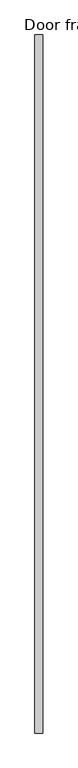
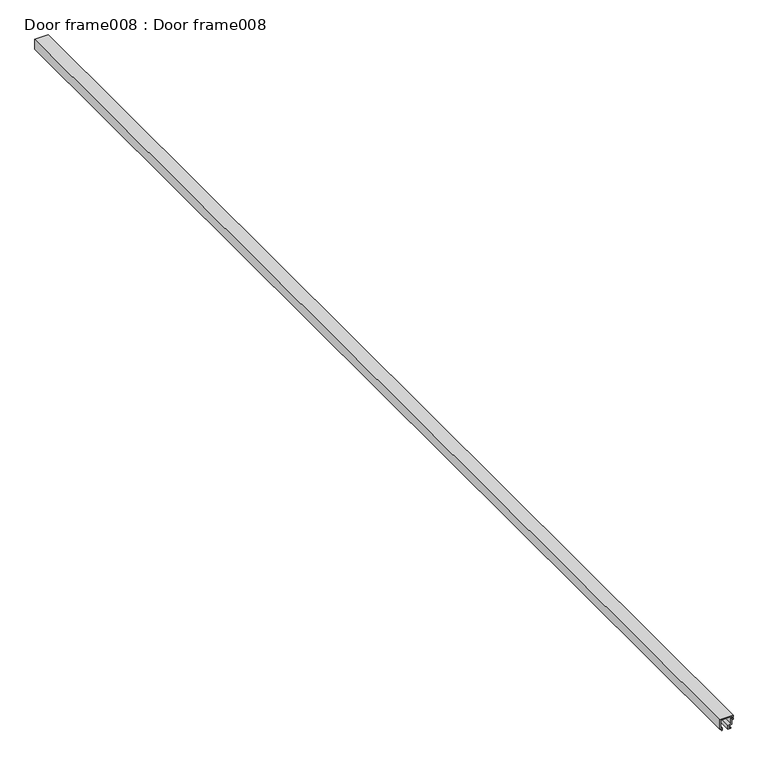
"""IFC4 building model written with IfcOpenShell, lengths in millimetres: proxy geometry, Door frame008 : Door frame008."""

import ifcopenshell
import ifcopenshell.guid

model = None  # the IFC model being written
_history = None  # IfcOwnerHistory: only IFC2X3 demands one
_inside = {}  # id of a spatial element -> (the spatial element, [elements in it])
_under = {}  # id of a project, library or spatial element -> (it, [spatial elements below it])
_declared = {}  # id of a project -> (the project, [libraries it declares])
_typed = {}  # id of a type object -> (the type object, [elements of that type])
_made_of = {}  # id of a material, layer set ... -> (it, [elements and type objects made of it])


def new_model(schema):
    """Start an empty IFC model of exactly this schema.

    Asked for "IFC4X3", IfcOpenShell would pick the latest addendum, in which some entities
    have other attributes; the version numbers below select the first issue.
    IFC2X3 requires an IfcOwnerHistory on every rooted entity: one is made here for all.
    """
    global model, _history
    if schema == "IFC4X3":
        model = ifcopenshell.file(schema_version=(4, 3, 0, 0))
    else:
        model = ifcopenshell.file(schema=schema)
    _inside.clear()
    _under.clear()
    _declared.clear()
    _typed.clear()
    _made_of.clear()
    _history = None
    if model.schema == "IFC2X3":
        org = make("IfcOrganization", Name="unknown")
        user = make(
            "IfcPersonAndOrganization",
            ThePerson=make("IfcPerson", FamilyName="unknown"),
            TheOrganization=org,
        )
        app = make(
            "IfcApplication",
            ApplicationDeveloper=org,
            Version="unknown",
            ApplicationFullName="unknown",
            ApplicationIdentifier="unknown",
        )
        _history = make(
            "IfcOwnerHistory",
            OwningUser=user,
            OwningApplication=app,
            ChangeAction="ADDED",
            CreationDate=0,
        )
    return model


def make(cls, **values):
    """One entity of the class cls with the attributes given. An attribute that is None is left unset."""
    return model.create_entity(
        cls, **{name: value for name, value in values.items() if value is not None}
    )


def rooted(cls, **values):
    """An entity with a GlobalId (a new one), such as an element, a storey or a relation."""
    return make(cls, GlobalId=ifcopenshell.guid.new(), OwnerHistory=_history, **values)


def si_unit(unit_type, name, prefix=None):
    """IfcSIUnit, for example si_unit("LENGTHUNIT", "METRE", prefix="MILLI")."""
    return make("IfcSIUnit", UnitType=unit_type, Prefix=prefix, Name=name)


def assignment(units):
    """IfcUnitAssignment: the units of a project."""
    return None if units is None else make("IfcUnitAssignment", Units=units)


def point(xyz):
    """IfcCartesianPoint."""
    return None if xyz is None else make("IfcCartesianPoint", Coordinates=xyz)


def direction(xyz):
    """IfcDirection."""
    return None if xyz is None else make("IfcDirection", DirectionRatios=xyz)


def frame(location, z_axis=None, x_axis=None):
    """IfcAxis2Placement3D, a coordinate frame: its origin and axes. An axis left out is left unset."""
    return make(
        "IfcAxis2Placement3D",
        Location=point(location),
        Axis=direction(z_axis),
        RefDirection=direction(x_axis),
    )


def origin():
    """The frame at (0, 0, 0) with its axes left unset."""
    return frame((0.0, 0.0, 0.0))


def place(relative_to, where):
    """IfcLocalPlacement: puts the frame where relative to a parent placement (None: the world)."""
    return make(
        "IfcLocalPlacement", PlacementRelTo=relative_to, RelativePlacement=where
    )


def context(
    kind, dimensions, precision=None, world=None, true_north=None, identifier=None
):
    """IfcGeometricRepresentationContext, for example the 3D "Model" context."""
    return make(
        "IfcGeometricRepresentationContext",
        ContextIdentifier=identifier,
        ContextType=kind,
        CoordinateSpaceDimension=dimensions,
        Precision=precision,
        WorldCoordinateSystem=world,
        TrueNorth=true_north,
    )


def project(units=None, contexts=None):
    """IfcProject with its units and contexts."""
    return rooted(
        "IfcProject",
        Name="project",
        RepresentationContexts=contexts,
        UnitsInContext=assignment(units),
    )


def spatial(cls, under=None, at=None, **own):
    """A site, building, storey or space (cls), placed at a placement, below another one or the project."""
    s = rooted(cls, ObjectPlacement=at, **own)
    if under is not None:
        _under.setdefault(under.id(), (under, []))[1].append(s)
    return s


def polyline(points):
    """IfcPolyline through the points."""
    return make("IfcPolyline", Points=[point(p) for p in points])


def outline(outer, holes=None, kind="AREA"):
    """IfcArbitraryClosedProfileDef: a profile drawn as a closed curve; with holes, ...WithVoids."""
    if holes is None:
        return make("IfcArbitraryClosedProfileDef", ProfileType=kind, OuterCurve=outer)
    return make(
        "IfcArbitraryProfileDefWithVoids",
        ProfileType=kind,
        OuterCurve=outer,
        InnerCurves=holes,
    )


def extrude(swept, where, along, depth):
    """IfcExtrudedAreaSolid: the profile swept, set in the frame where, extruded along a direction by depth."""
    return make(
        "IfcExtrudedAreaSolid",
        SweptArea=swept,
        Position=where,
        ExtrudedDirection=direction(along),
        Depth=depth,
    )


def shape(context_of_items, identifier, shape_type, items):
    """IfcShapeRepresentation: the items that make up one representation, for example the "Body"."""
    return make(
        "IfcShapeRepresentation",
        ContextOfItems=context_of_items,
        RepresentationIdentifier=identifier,
        RepresentationType=shape_type,
        Items=items,
    )


def source(mapping_origin, context_of_items, identifier, shape_type, items):
    """IfcRepresentationMap: a shape defined once, which mapped items show again and again."""
    return make(
        "IfcRepresentationMap",
        MappingOrigin=mapping_origin,
        MappedRepresentation=shape(context_of_items, identifier, shape_type, items),
    )


def transform(
    local_origin,
    x_axis=None,
    y_axis=None,
    z_axis=None,
    scale=None,
    scale2=None,
    scale3=None,
    uniform=True,
):
    """IfcCartesianTransformationOperator3D, or its non-uniform kind. x_axis, y_axis, z_axis: its Axis1, 2, 3."""
    if uniform:
        return make(
            "IfcCartesianTransformationOperator3D",
            Axis1=direction(x_axis),
            Axis2=direction(y_axis),
            LocalOrigin=point(local_origin),
            Scale=scale,
            Axis3=direction(z_axis),
        )
    return make(
        "IfcCartesianTransformationOperator3DnonUniform",
        Axis1=direction(x_axis),
        Axis2=direction(y_axis),
        LocalOrigin=point(local_origin),
        Scale=scale,
        Axis3=direction(z_axis),
        Scale2=scale2,
        Scale3=scale3,
    )


def mapped(mapping_source, mapping_target):
    """IfcMappedItem: shows the shape of a source again, moved by a transform."""
    return make(
        "IfcMappedItem", MappingSource=mapping_source, MappingTarget=mapping_target
    )


def made_of(thing, what):
    """Note that an element or type object is made of a material, layer set ...; save() writes the relation."""
    if what is not None:
        _made_of.setdefault(what.id(), (what, []))[1].append(thing)
    return thing


def element(
    cls,
    number,
    at=None,
    inside=None,
    cuts=None,
    type_object=None,
    material=None,
    context=None,
    identifier="Body",
    shape_type=None,
    held_by="IfcProductDefinitionShape",
    body=None,
    shapes=None,
    **own,
):
    """One element of the class cls, such as IfcWall. Its Tag is "e" and its number.

    at: its placement. inside: the storey or other place that contains it. cuts: it is an
    opening in that element (IfcRelVoidsElement). A single representation is given by context,
    identifier, shape_type and body (its items); several are given by shapes. held_by: the class
    of the entity that holds the representations. save() writes the other relations.
    """
    e = rooted(cls, Tag="e%d" % number, ObjectPlacement=at, **own)
    if body is not None:
        shapes = [shape(context, identifier, shape_type, body)]
    if shapes is not None:
        e.Representation = make(held_by, Representations=shapes)
    if inside is not None:
        _inside.setdefault(inside.id(), (inside, []))[1].append(e)
    if cuts is not None:
        rooted(
            "IfcRelVoidsElement", RelatingBuildingElement=cuts, RelatedOpeningElement=e
        )
    if type_object is not None:
        _typed.setdefault(type_object.id(), (type_object, []))[1].append(e)
    return made_of(e, material)


def aggregate(whole, parts):
    """IfcRelAggregates: a whole, such as a stair, and the parts it consists of."""
    return rooted("IfcRelAggregates", RelatingObject=whole, RelatedObjects=parts)


def save(model, path):
    """Write the relations noted so far, then the file.

    IfcRelAggregates (storeys below a building ...), IfcRelContainedInSpatialStructure (elements
    in a storey), IfcRelDefinesByType, IfcRelAssociatesMaterial and IfcRelDeclares: one each for
    every whole, place, type object, material and project.
    """
    for whole, parts in _under.values():
        aggregate(whole, parts)
    for where, things in _inside.values():
        rooted(
            "IfcRelContainedInSpatialStructure",
            RelatedElements=things,
            RelatingStructure=where,
        )
    for kind, things in _typed.values():
        rooted("IfcRelDefinesByType", RelatedObjects=things, RelatingType=kind)
    for what, things in _made_of.values():
        rooted("IfcRelAssociatesMaterial", RelatedObjects=things, RelatingMaterial=what)
    for by, libraries in _declared.values():
        rooted("IfcRelDeclares", RelatingContext=by, RelatedDefinitions=libraries)
    model.write(path)


def door_frame008_door_frame008_4371c8f4(model_context):
    return source(origin(), model_context, "Body", "SweptSolid", [
        extrude(outline(polyline([(36665.0550947, 15518.5928473), (36665.0550947, 15523.2947939), (36666.4520947, 15523.2947939), (36666.4520947, 15520.1676473), (36670.1011414, 15520.1676473), (36671.9000345, 15524.8924515), (36679.2790947, 15524.8924515), (36679.2790947, 15527.4324515), (36681.9249044, 15527.4324515), (36681.9249044, 15526.1777759), (36680.6298938, 15526.1777759), (36680.6298938, 15524.6927561), (36685.5545864, 15524.6927561), (36685.5545864, 15526.1777759), (36684.2230088, 15526.1777759), (36684.2230088, 15527.4324515), (36686.8990947, 15527.4324515), (36686.8990947, 15504.8264515), (36669.5427612, 15504.8264515), (36669.5427612, 15507.7728515), (36668.8374665, 15508.1726577), (36667.4225662, 15507.3557647), (36666.0872218, 15508.6911091), (36666.4062067, 15509.5508515), (36670.8462947, 15509.5508515), (36670.8462947, 15506.2234515), (36685.5020947, 15506.2234515), (36685.5020947, 15523.4954515), (36673.0532282, 15523.4954515), (36671.1866406, 15518.5928473), (36665.0550947, 15518.5928473)])), frame((0.0, -1052.8906567, 0.0), z_axis=(0.0, 1.0, 0.0), x_axis=(0.0, 0.0, 1.0)), (0.0, 0.0, 1.0), 1999.85),
    ])


if __name__ == "__main__":
    model = new_model("IFC4")
    model_context = context("Model", 3, world=origin())
    ifc_project = project(units=[si_unit("LENGTHUNIT", "METRE", prefix="MILLI")], contexts=[model_context])
    site = spatial("IfcSite", under=ifc_project)
    building = spatial("IfcBuilding", under=site)
    placement = place(None, origin())
    door_frame008_door_frame008_shape = door_frame008_door_frame008_4371c8f4(model_context)
    element("IfcBuildingElementProxy", 1, Name="Door frame008 : Door frame008", ObjectType="Door frame008 : Door frame008", at=placement, inside=building, context=model_context, shape_type="MappedRepresentation", body=[
        mapped(door_frame008_door_frame008_shape, transform((0.0, 0.0, 0.0), x_axis=(1.0, 0.0, 0.0), y_axis=(0.0, 1.0, 0.0), z_axis=(0.0, 0.0, 1.0))),
    ])
    save(model, "model.ifc")

# Revit data of these elements
# Type "Door frame008 : Door frame008"
#   NameOverride = "Door frame008"
# Element 1 (IfcBuildingElementProxy, "Door frame008 : Door frame008")
#   Materials on its faces: "FLEETWOOD SERIES T-3200 SINGLE SWING DOOR FRAME"
# Materials
#   "FLEETWOOD SERIES T-3200 SINGLE SWING DOOR FRAME": class "Unassigned", colour RGB 128 128 128, transparency 0, Cost = 0
